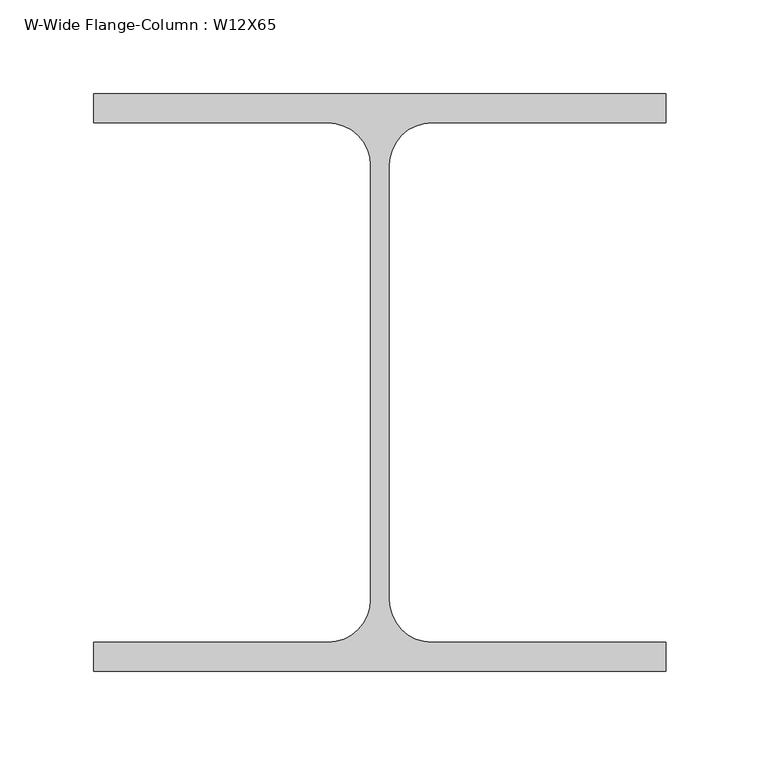
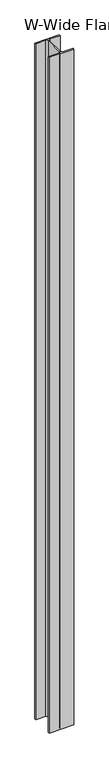
"""IFC4 building model written with IfcOpenShell, lengths in millimetres: column geometry, W-Wide Flange-Column : W12X65."""

from ifc_helpers import new_model, si_unit, point, frame, frame_2d, origin, place, context, project, spatial, polyline, circle_curve, trimmed, segment, composite_curve, outline, extrude, source, transform, mapped, element, save


def w_wide_flange_column_w12x65_febec582(model_context):
    return source(origin(), model_context, "Body", "SweptSolid", [
        extrude(outline(composite_curve([segment(polyline([(152.4, 153.67), (152.4, 138.303), (27.686, 138.303)]), True, "CONTINUOUS"), segment(trimmed(circle_curve(frame_2d((27.686, 115.57)), 22.733), [point((27.686, 138.303))], [point((4.953, 115.57))], True, "CARTESIAN"), True, "CONTINUOUS"), segment(polyline([(4.953, 115.57), (4.953, -115.57)]), True, "CONTINUOUS"), segment(trimmed(circle_curve(frame_2d((27.686, -115.57)), 22.733), [point((4.953, -115.57))], [point((27.686, -138.303))], True, "CARTESIAN"), True, "CONTINUOUS"), segment(polyline([(27.686, -138.303), (152.4, -138.303), (152.4, -153.67), (-152.4, -153.67), (-152.4, -138.303), (-27.686, -138.303)]), True, "CONTINUOUS"), segment(trimmed(circle_curve(frame_2d((-27.686, -115.57)), 22.733), [point((-27.686, -138.303))], [point((-4.953, -115.57))], True, "CARTESIAN"), True, "CONTINUOUS"), segment(polyline([(-4.953, -115.57), (-4.953, 115.57)]), True, "CONTINUOUS"), segment(trimmed(circle_curve(frame_2d((-27.686, 115.57)), 22.733), [point((-4.953, 115.57))], [point((-27.686, 138.303))], True, "CARTESIAN"), True, "CONTINUOUS"), segment(polyline([(-27.686, 138.303), (-152.4, 138.303), (-152.4, 153.67), (152.4, 153.67)]), True, "CONTINUOUS")], self_intersect=False)), frame((0.0, 0.0, 8756.65), z_axis=(0.0, 0.0, 1.0), x_axis=(1.0, 0.0, 0.0)), (0.0, 0.0, 1.0), 8870.95),
    ])


if __name__ == "__main__":
    model = new_model("IFC4")
    model_context = context("Model", 3, world=origin())
    ifc_project = project(units=[si_unit("LENGTHUNIT", "METRE", prefix="MILLI")], contexts=[model_context])
    site = spatial("IfcSite", under=ifc_project)
    building = spatial("IfcBuilding", under=site)
    placement = place(None, origin())
    w_wide_flange_column_w12x65_shape = w_wide_flange_column_w12x65_febec582(model_context)
    element("IfcColumn", 1, ObjectType="W-Wide Flange-Column : W12X65", at=placement, inside=building, context=model_context, shape_type="MappedRepresentation", body=[
        mapped(w_wide_flange_column_w12x65_shape, transform((0.0, 0.0, 0.0), x_axis=(1.0, 0.0, 0.0), y_axis=(0.0, 1.0, 0.0), z_axis=(0.0, 0.0, 1.0))),
    ])
    save(model, "model.ifc")

# Revit data of these elements
# Type "W-Wide Flange-Column : W12X65"
#   Assembly Code = "B10"
#   W = 65
#   bf = 1' - 0"
#   d = 1' - 0.1"
#   k = 0' - 1 1/2"
#   kr = 0' - 0.895"
#   tf = 0' - 0.605"
#   tw = 0' - 0.39"
#   A = 0.132639 SF
#   Structural Material [instance default] = Steel ASTM A992
# Element 1 (IfcColumn, "W-Wide Flange-Column : W12X65")
#   Materials on its faces: "Steel ASTM A992"
# Materials
#   "Steel ASTM A992": class "Metal", colour RGB 199 199 199, transparency 0, Description = "Structural steel 50ksi", Cost = 0
